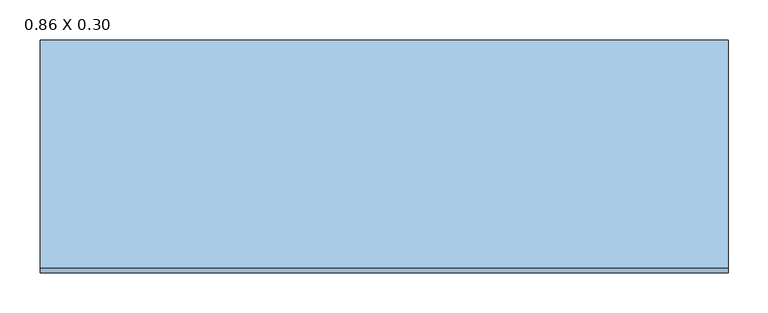
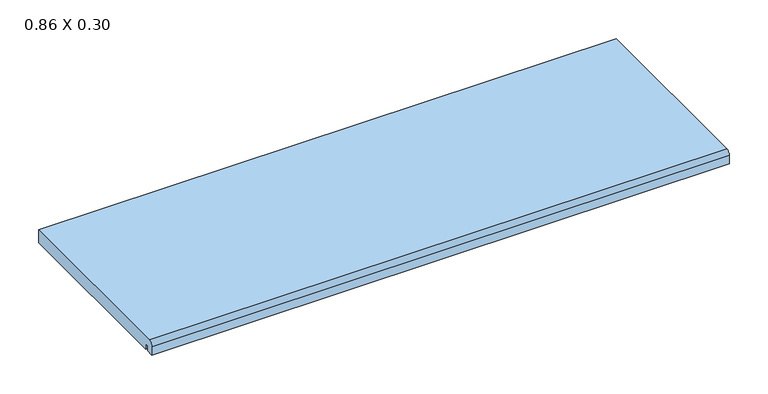
"""IFC4 building model written with IfcOpenShell, lengths in millimetres: window geometry, .CC_ND 300_PEDRA_PEITORIL RETO : 0.86 X 0.30."""

from ifc_helpers import new_model, si_unit, point, frame, frame_2d, origin, place, context, project, spatial, polyline, circle_curve, trimmed, segment, composite_curve, outline, extrude, source, transform, mapped, element, save


def window_0_86_x_0_30_12272b82(model_context):
    return source(origin(), model_context, "Body", "SweptSolid", [
        extrude(outline(composite_curve([segment(polyline([(-132.5083081, 1480.0), (-132.5083081, 1488.1993124), (-137.2619526, 1488.1993124), (-137.2619526, 1480.0), (-148.0, 1480.0), (-148.0, 1493.3808343)]), True, "CONTINUOUS"), segment(trimmed(circle_curve(frame_2d((-141.3808343, 1493.3808343)), 6.6191657), [point((-148.0, 1493.3808343))], [point((-141.3808343, 1500.0))], False, "CARTESIAN"), True, "CONTINUOUS"), segment(polyline([(-141.3808343, 1500.0), (143.7, 1500.0), (143.7, 1480.0), (-132.5083081, 1480.0)]), True, "CONTINUOUS")], self_intersect=False)), frame((-430.0, 0.0, 0.0), z_axis=(1.0, 0.0, 0.0), x_axis=(0.0, 1.0, 0.0)), (0.0, 0.0, 1.0), 860.0),
    ])


if __name__ == "__main__":
    model = new_model("IFC4")
    model_context = context("Model", 3, world=origin())
    ifc_project = project(units=[si_unit("LENGTHUNIT", "METRE", prefix="MILLI")], contexts=[model_context])
    site = spatial("IfcSite", under=ifc_project)
    building = spatial("IfcBuilding", under=site)
    placement = place(None, origin())
    window_0_86_x_0_30_shape = window_0_86_x_0_30_12272b82(model_context)
    element("IfcWindow", 1, ObjectType=".CC_ND 300_PEDRA_PEITORIL RETO : 0.86 X 0.30", at=placement, inside=building, context=model_context, shape_type="MappedRepresentation", body=[
        mapped(window_0_86_x_0_30_shape, transform((0.0, 0.0, 0.0), x_axis=(1.0, 0.0, 0.0), y_axis=(0.0, 1.0, 0.0), z_axis=(0.0, 0.0, 1.0))),
    ])
    save(model, "model.ifc")

# Revit data of these elements
# Type ".CC_ND 300_PEDRA_PEITORIL RETO : 0.86 X 0.30"
#   Type Mark = "66"
#   Largura da pedra [instance default] = 0.26 m
#   Extensão interior peitoril [instance default] = 0.03 m
#   Extensão exterior peitoril [instance default] = 0.03 m
#   Espessura = 0.02 m
#   Comprimento = 0.86 m
#   Altura-padrão do peitoril = 1.48 m
#   Peitoril = .GRANITO_BRANCO_ITAUNAS
#   Rough Width = 0
#   Rough Height = 0
#   Height = 0
#   Wall Closure = (empty or 0)
#   Width = 0
# Element 1 (IfcWindow, ".CC_ND 300_PEDRA_PEITORIL RETO : 0.86 X 0.30")
#   Largura da pedra = 0.2917 m
#   Extensão interior peitoril = 0.0257 m
#   Materials on its faces: ".GRANITO_BRANCO_ITAUNAS"
# Materials
#   ".GRANITO_BRANCO_ITAUNAS": class ".CC_PEDRA REVEST.", colour RGB 202 195 174, transparency 0, Description = "Revestimento em granito", Cost = 0
